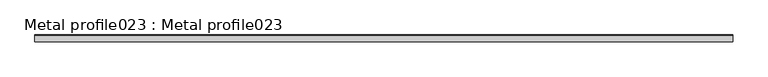
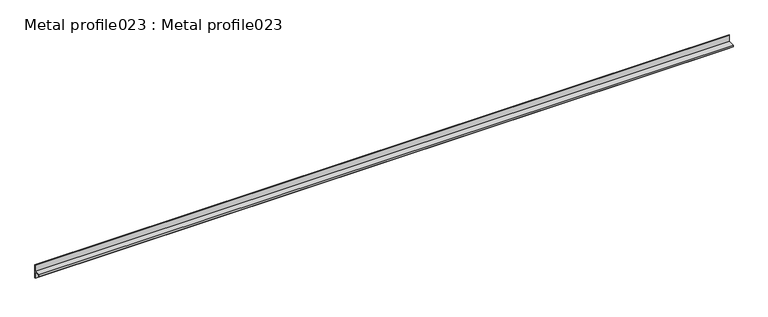
"""IFC4 building model written with IfcOpenShell, lengths in millimetres: proxy geometry, Metal profile023 : Metal profile023."""

import ifcopenshell
import ifcopenshell.guid

model = None  # the IFC model being written
_history = None  # IfcOwnerHistory: only IFC2X3 demands one
_inside = {}  # id of a spatial element -> (the spatial element, [elements in it])
_under = {}  # id of a project, library or spatial element -> (it, [spatial elements below it])
_declared = {}  # id of a project -> (the project, [libraries it declares])
_typed = {}  # id of a type object -> (the type object, [elements of that type])
_made_of = {}  # id of a material, layer set ... -> (it, [elements and type objects made of it])


def new_model(schema):
    """Start an empty IFC model of exactly this schema.

    Asked for "IFC4X3", IfcOpenShell would pick the latest addendum, in which some entities
    have other attributes; the version numbers below select the first issue.
    IFC2X3 requires an IfcOwnerHistory on every rooted entity: one is made here for all.
    """
    global model, _history
    if schema == "IFC4X3":
        model = ifcopenshell.file(schema_version=(4, 3, 0, 0))
    else:
        model = ifcopenshell.file(schema=schema)
    _inside.clear()
    _under.clear()
    _declared.clear()
    _typed.clear()
    _made_of.clear()
    _history = None
    if model.schema == "IFC2X3":
        org = make("IfcOrganization", Name="unknown")
        user = make(
            "IfcPersonAndOrganization",
            ThePerson=make("IfcPerson", FamilyName="unknown"),
            TheOrganization=org,
        )
        app = make(
            "IfcApplication",
            ApplicationDeveloper=org,
            Version="unknown",
            ApplicationFullName="unknown",
            ApplicationIdentifier="unknown",
        )
        _history = make(
            "IfcOwnerHistory",
            OwningUser=user,
            OwningApplication=app,
            ChangeAction="ADDED",
            CreationDate=0,
        )
    return model


def make(cls, **values):
    """One entity of the class cls with the attributes given. An attribute that is None is left unset."""
    return model.create_entity(
        cls, **{name: value for name, value in values.items() if value is not None}
    )


def rooted(cls, **values):
    """An entity with a GlobalId (a new one), such as an element, a storey or a relation."""
    return make(cls, GlobalId=ifcopenshell.guid.new(), OwnerHistory=_history, **values)


def si_unit(unit_type, name, prefix=None):
    """IfcSIUnit, for example si_unit("LENGTHUNIT", "METRE", prefix="MILLI")."""
    return make("IfcSIUnit", UnitType=unit_type, Prefix=prefix, Name=name)


def assignment(units):
    """IfcUnitAssignment: the units of a project."""
    return None if units is None else make("IfcUnitAssignment", Units=units)


def point(xyz):
    """IfcCartesianPoint."""
    return None if xyz is None else make("IfcCartesianPoint", Coordinates=xyz)


def direction(xyz):
    """IfcDirection."""
    return None if xyz is None else make("IfcDirection", DirectionRatios=xyz)


def frame(location, z_axis=None, x_axis=None):
    """IfcAxis2Placement3D, a coordinate frame: its origin and axes. An axis left out is left unset."""
    return make(
        "IfcAxis2Placement3D",
        Location=point(location),
        Axis=direction(z_axis),
        RefDirection=direction(x_axis),
    )


def origin():
    """The frame at (0, 0, 0) with its axes left unset."""
    return frame((0.0, 0.0, 0.0))


def place(relative_to, where):
    """IfcLocalPlacement: puts the frame where relative to a parent placement (None: the world)."""
    return make(
        "IfcLocalPlacement", PlacementRelTo=relative_to, RelativePlacement=where
    )


def context(
    kind, dimensions, precision=None, world=None, true_north=None, identifier=None
):
    """IfcGeometricRepresentationContext, for example the 3D "Model" context."""
    return make(
        "IfcGeometricRepresentationContext",
        ContextIdentifier=identifier,
        ContextType=kind,
        CoordinateSpaceDimension=dimensions,
        Precision=precision,
        WorldCoordinateSystem=world,
        TrueNorth=true_north,
    )


def project(units=None, contexts=None):
    """IfcProject with its units and contexts."""
    return rooted(
        "IfcProject",
        Name="project",
        RepresentationContexts=contexts,
        UnitsInContext=assignment(units),
    )


def spatial(cls, under=None, at=None, **own):
    """A site, building, storey or space (cls), placed at a placement, below another one or the project."""
    s = rooted(cls, ObjectPlacement=at, **own)
    if under is not None:
        _under.setdefault(under.id(), (under, []))[1].append(s)
    return s


def polyline(points):
    """IfcPolyline through the points."""
    return make("IfcPolyline", Points=[point(p) for p in points])


def outline(outer, holes=None, kind="AREA"):
    """IfcArbitraryClosedProfileDef: a profile drawn as a closed curve; with holes, ...WithVoids."""
    if holes is None:
        return make("IfcArbitraryClosedProfileDef", ProfileType=kind, OuterCurve=outer)
    return make(
        "IfcArbitraryProfileDefWithVoids",
        ProfileType=kind,
        OuterCurve=outer,
        InnerCurves=holes,
    )


def extrude(swept, where, along, depth):
    """IfcExtrudedAreaSolid: the profile swept, set in the frame where, extruded along a direction by depth."""
    return make(
        "IfcExtrudedAreaSolid",
        SweptArea=swept,
        Position=where,
        ExtrudedDirection=direction(along),
        Depth=depth,
    )


def shape(context_of_items, identifier, shape_type, items):
    """IfcShapeRepresentation: the items that make up one representation, for example the "Body"."""
    return make(
        "IfcShapeRepresentation",
        ContextOfItems=context_of_items,
        RepresentationIdentifier=identifier,
        RepresentationType=shape_type,
        Items=items,
    )


def source(mapping_origin, context_of_items, identifier, shape_type, items):
    """IfcRepresentationMap: a shape defined once, which mapped items show again and again."""
    return make(
        "IfcRepresentationMap",
        MappingOrigin=mapping_origin,
        MappedRepresentation=shape(context_of_items, identifier, shape_type, items),
    )


def transform(
    local_origin,
    x_axis=None,
    y_axis=None,
    z_axis=None,
    scale=None,
    scale2=None,
    scale3=None,
    uniform=True,
):
    """IfcCartesianTransformationOperator3D, or its non-uniform kind. x_axis, y_axis, z_axis: its Axis1, 2, 3."""
    if uniform:
        return make(
            "IfcCartesianTransformationOperator3D",
            Axis1=direction(x_axis),
            Axis2=direction(y_axis),
            LocalOrigin=point(local_origin),
            Scale=scale,
            Axis3=direction(z_axis),
        )
    return make(
        "IfcCartesianTransformationOperator3DnonUniform",
        Axis1=direction(x_axis),
        Axis2=direction(y_axis),
        LocalOrigin=point(local_origin),
        Scale=scale,
        Axis3=direction(z_axis),
        Scale2=scale2,
        Scale3=scale3,
    )


def mapped(mapping_source, mapping_target):
    """IfcMappedItem: shows the shape of a source again, moved by a transform."""
    return make(
        "IfcMappedItem", MappingSource=mapping_source, MappingTarget=mapping_target
    )


def made_of(thing, what):
    """Note that an element or type object is made of a material, layer set ...; save() writes the relation."""
    if what is not None:
        _made_of.setdefault(what.id(), (what, []))[1].append(thing)
    return thing


def element(
    cls,
    number,
    at=None,
    inside=None,
    cuts=None,
    type_object=None,
    material=None,
    context=None,
    identifier="Body",
    shape_type=None,
    held_by="IfcProductDefinitionShape",
    body=None,
    shapes=None,
    **own,
):
    """One element of the class cls, such as IfcWall. Its Tag is "e" and its number.

    at: its placement. inside: the storey or other place that contains it. cuts: it is an
    opening in that element (IfcRelVoidsElement). A single representation is given by context,
    identifier, shape_type and body (its items); several are given by shapes. held_by: the class
    of the entity that holds the representations. save() writes the other relations.
    """
    e = rooted(cls, Tag="e%d" % number, ObjectPlacement=at, **own)
    if body is not None:
        shapes = [shape(context, identifier, shape_type, body)]
    if shapes is not None:
        e.Representation = make(held_by, Representations=shapes)
    if inside is not None:
        _inside.setdefault(inside.id(), (inside, []))[1].append(e)
    if cuts is not None:
        rooted(
            "IfcRelVoidsElement", RelatingBuildingElement=cuts, RelatedOpeningElement=e
        )
    if type_object is not None:
        _typed.setdefault(type_object.id(), (type_object, []))[1].append(e)
    return made_of(e, material)


def aggregate(whole, parts):
    """IfcRelAggregates: a whole, such as a stair, and the parts it consists of."""
    return rooted("IfcRelAggregates", RelatingObject=whole, RelatedObjects=parts)


def save(model, path):
    """Write the relations noted so far, then the file.

    IfcRelAggregates (storeys below a building ...), IfcRelContainedInSpatialStructure (elements
    in a storey), IfcRelDefinesByType, IfcRelAssociatesMaterial and IfcRelDeclares: one each for
    every whole, place, type object, material and project.
    """
    for whole, parts in _under.values():
        aggregate(whole, parts)
    for where, things in _inside.values():
        rooted(
            "IfcRelContainedInSpatialStructure",
            RelatedElements=things,
            RelatingStructure=where,
        )
    for kind, things in _typed.values():
        rooted("IfcRelDefinesByType", RelatedObjects=things, RelatingType=kind)
    for what, things in _made_of.values():
        rooted("IfcRelAssociatesMaterial", RelatedObjects=things, RelatingMaterial=what)
    for by, libraries in _declared.values():
        rooted("IfcRelDeclares", RelatingContext=by, RelatedDefinitions=libraries)
    model.write(path)


def metal_profile023_metal_profile023_a1b0dacf(model_context):
    return source(origin(), model_context, "Body", "SweptSolid", [
        extrude(outline(polyline([(-4684.6182816, 39565.1268195), (-4684.6182816, 39561.6470195), (-4685.8882816, 39561.6470195), (-4685.8882816, 39566.3968195), (-4667.6543336, 39566.3968195), (-4667.6543336, 39585.4468195), (-4666.3843336, 39585.4468195), (-4666.3843336, 39546.0768195), (-4667.6543336, 39546.0768195), (-4667.6543336, 39565.1268195), (-4684.6182816, 39565.1268195)])), frame((12383.0178845, 0.0, 0.0), z_axis=(1.0, 0.0, 0.0), x_axis=(0.0, 1.0, 0.0)), (0.0, 0.0, 1.0), 2000.0),
    ])


if __name__ == "__main__":
    model = new_model("IFC4")
    model_context = context("Model", 3, world=origin())
    ifc_project = project(units=[si_unit("LENGTHUNIT", "METRE", prefix="MILLI")], contexts=[model_context])
    site = spatial("IfcSite", under=ifc_project)
    building = spatial("IfcBuilding", under=site)
    placement = place(None, origin())
    metal_profile023_metal_profile023_shape = metal_profile023_metal_profile023_a1b0dacf(model_context)
    element("IfcBuildingElementProxy", 1, Name="Metal profile023 : Metal profile023", ObjectType="Metal profile023 : Metal profile023", at=placement, inside=building, context=model_context, shape_type="MappedRepresentation", body=[
        mapped(metal_profile023_metal_profile023_shape, transform((0.0, 0.0, 0.0), x_axis=(1.0, 0.0, 0.0), y_axis=(0.0, 1.0, 0.0), z_axis=(0.0, 0.0, 1.0))),
    ])
    save(model, "model.ifc")

# Revit data of these elements
# Type "Metal profile023 : Metal profile023"
#   NameOverride = "Metal profile023"
# Element 1 (IfcBuildingElementProxy, "Metal profile023 : Metal profile023")
#   Materials on its faces: "16 GA. COPPER VENTED T REVEAL BEAD"
# Materials
#   "16 GA. COPPER VENTED T REVEAL BEAD": class "Unassigned", colour RGB 255 227 10, transparency 0
